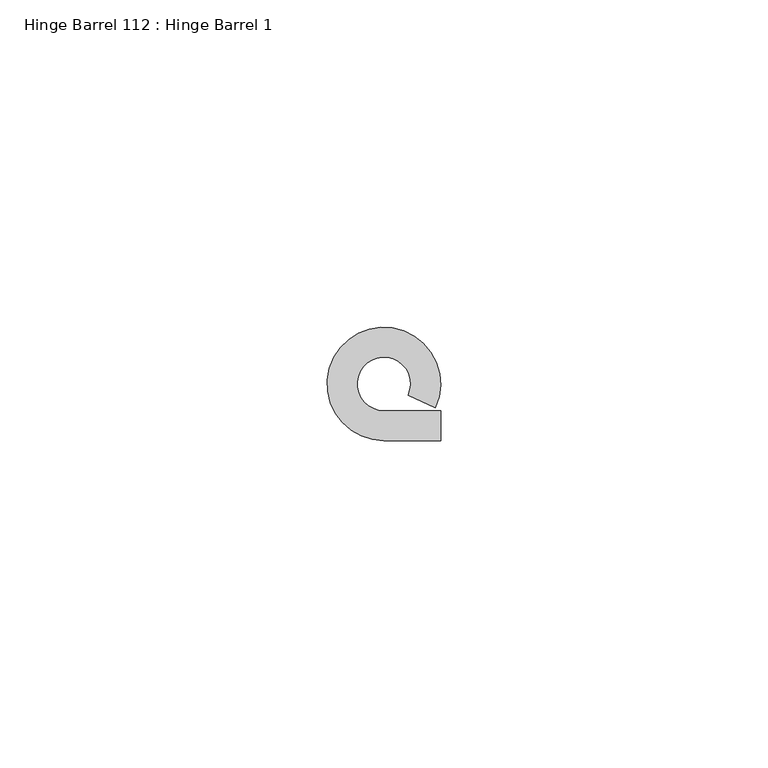
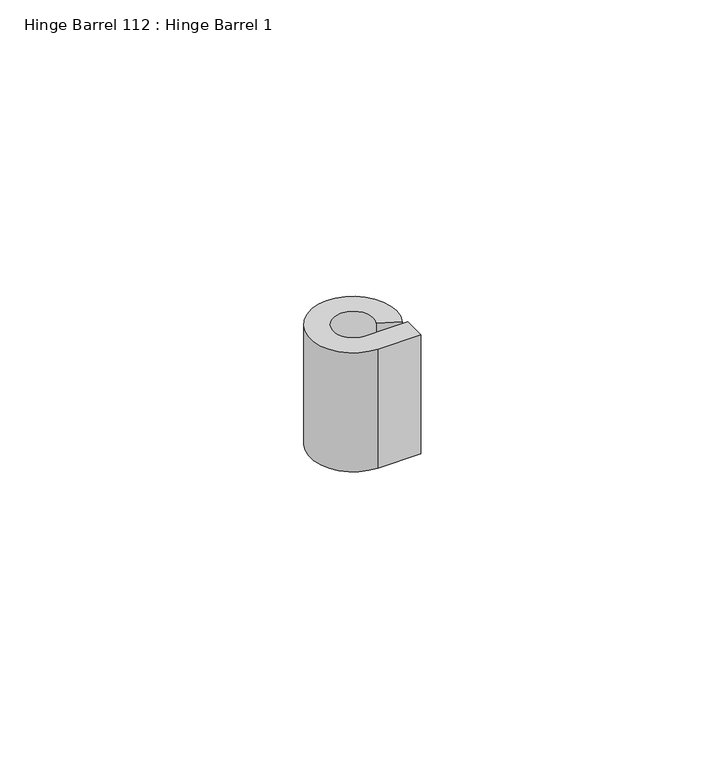
"""IFC4 building model written with IfcOpenShell, lengths in millimetres: proxy geometry, Hinge Barrel 112 : Hinge Barrel 1."""

from ifc_helpers import new_model, si_unit, point, frame, frame_2d, origin, place, context, project, spatial, polyline, circle_curve, trimmed, segment, composite_curve, outline, extrude, source, transform, mapped, element, save


def hinge_barrel_112_hinge_barrel_1_a2f6928c(model_context):
    return source(origin(), model_context, "Body", "SweptSolid", [
        extrude(outline(composite_curve([segment(polyline([(587323.2214739, -534104.7943841), (587327.7934739, -534104.7943841), (587327.7934739, -534109.3584466), (587319.1320739, -534109.3584466)]), True, "CONTINUOUS"), segment(trimmed(circle_curve(frame_2d((587319.1320739, -534100.7049841)), 8.6534625), [point((587319.1320739, -534109.3584466))], [point((587326.986084, -534104.3377433))], False, "CARTESIAN"), True, "CONTINUOUS"), segment(polyline([(587326.986084, -534104.3377433), (587322.8436736, -534102.421731)]), True, "CONTINUOUS"), segment(trimmed(circle_curve(frame_2d((587319.1320739, -534100.7049841)), 4.0894), [point((587322.8436736, -534102.421731))], [point((587319.1320739, -534104.7943841))], True, "CARTESIAN"), True, "CONTINUOUS"), segment(polyline([(587319.1320739, -534104.7943841), (587323.2214739, -534104.7943841)]), True, "CONTINUOUS")], self_intersect=False)), frame((0.0, 0.0, 412.75), z_axis=(0.0, 0.0, 1.0), x_axis=(1.0, 0.0, 0.0)), (0.0, 0.0, 1.0), 25.4),
    ])


if __name__ == "__main__":
    model = new_model("IFC4")
    model_context = context("Model", 3, world=origin())
    ifc_project = project(units=[si_unit("LENGTHUNIT", "METRE", prefix="MILLI")], contexts=[model_context])
    site = spatial("IfcSite", under=ifc_project)
    building = spatial("IfcBuilding", under=site)
    placement = place(None, origin())
    hinge_barrel_112_hinge_barrel_1_shape = hinge_barrel_112_hinge_barrel_1_a2f6928c(model_context)
    element("IfcBuildingElementProxy", 1, Name="Hinge Barrel 112 : Hinge Barrel 1", ObjectType="Hinge Barrel 112 : Hinge Barrel 1", at=placement, inside=building, context=model_context, shape_type="MappedRepresentation", body=[
        mapped(hinge_barrel_112_hinge_barrel_1_shape, transform((0.0, 0.0, 0.0), x_axis=(1.0, 0.0, 0.0), y_axis=(0.0, 1.0, 0.0), z_axis=(0.0, 0.0, 1.0))),
    ])
    save(model, "model.ifc")

# Revit data of these elements
# Element 1 (IfcBuildingElementProxy, "Hinge Barrel 112 : Hinge Barrel 1")
#   Materials on its faces: "6\"X6\" WELD-ON STL BUTT HINGE"
# Materials
#   "6\"X6\" WELD-ON STL BUTT HINGE": class "Metal", colour RGB 189 187 185, transparency 0, Description = "Carbon steel", Cost = 0
